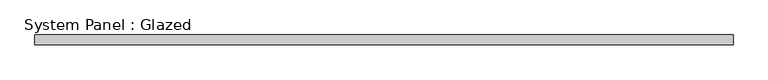
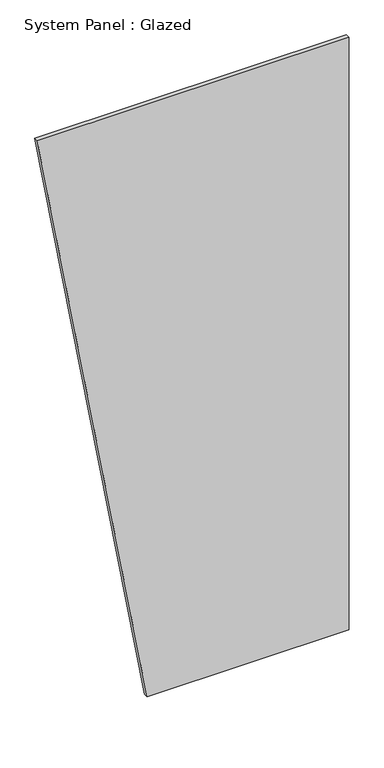
"""IFC4 building model written with IfcOpenShell, lengths in millimetres: plate geometry, System Panel : Glazed."""

from ifc_helpers import new_model, si_unit, frame, origin, place, context, project, spatial, polyline, outline, extrude, source, transform, mapped, element, save


def system_panel_glazed_e7bd2299(model_context):
    return source(origin(), model_context, "Body", "SweptSolid", [
        extrude(outline(polyline([(0.0, -268.2393521), (0.0, 910.7187498), (3657.6, 910.7187498), (3657.6, -910.7187498), (0.0, -268.2393521)])), frame((0.0, -44.45, 0.0), z_axis=(0.0, 1.0, 0.0), x_axis=(0.0, 0.0, 1.0)), (0.0, 0.0, 1.0), 25.4),
    ])


if __name__ == "__main__":
    model = new_model("IFC4")
    model_context = context("Model", 3, world=origin())
    ifc_project = project(units=[si_unit("LENGTHUNIT", "METRE", prefix="MILLI")], contexts=[model_context])
    site = spatial("IfcSite", under=ifc_project)
    building = spatial("IfcBuilding", under=site)
    placement = place(None, origin())
    system_panel_glazed_shape = system_panel_glazed_e7bd2299(model_context)
    element("IfcPlate", 1, ObjectType="System Panel : Glazed", at=placement, inside=building, context=model_context, shape_type="MappedRepresentation", body=[
        mapped(system_panel_glazed_shape, transform((0.0, 0.0, 0.0), x_axis=(1.0, 0.0, 0.0), y_axis=(0.0, 1.0, 0.0), z_axis=(0.0, 0.0, 1.0))),
    ])
    save(model, "model.ifc")

# Revit data of these elements
# Type "System Panel : Glazed"
#   Construction Type Id = "GSP4R"
#   Analytic Construction = "1/8 in Pilkington single glazing"
#   Visual Light Transmittance = 0.9
#   Solar Heat Gain Coefficient = 0.86
#   Heat Transfer Coefficient (U) = 1.18115 BTU/(h·ft²·°F)
#   Define Thermal Properties by = 1
# Element 1 (IfcPlate, "System Panel : Glazed")
#   Materials on its faces: "Glass"
# Materials
#   "Glass": class "Glass", colour RGB 0 128 192, transparency 0.75, Description = "Soda Lime Glass", Cost = 0
